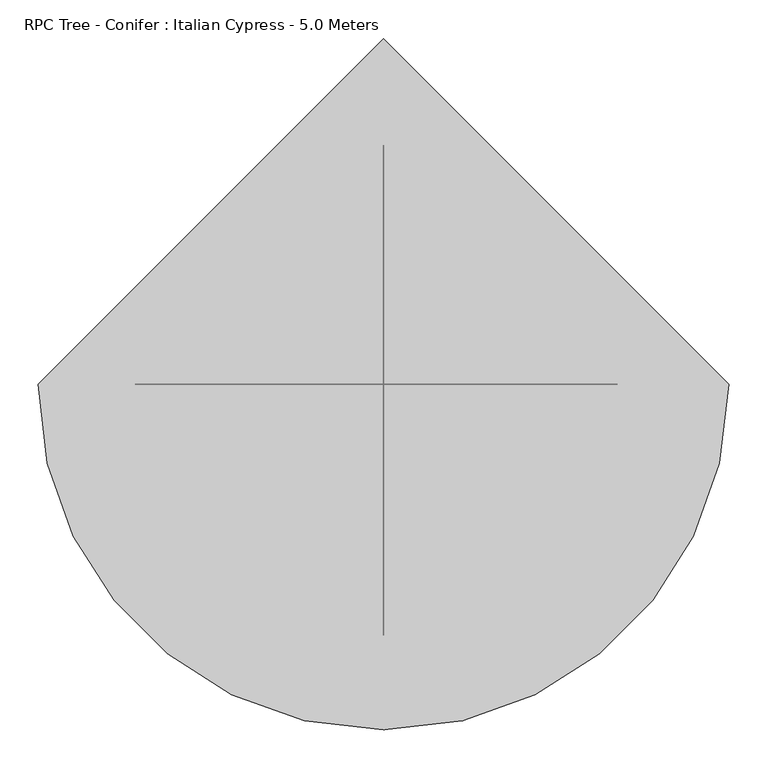
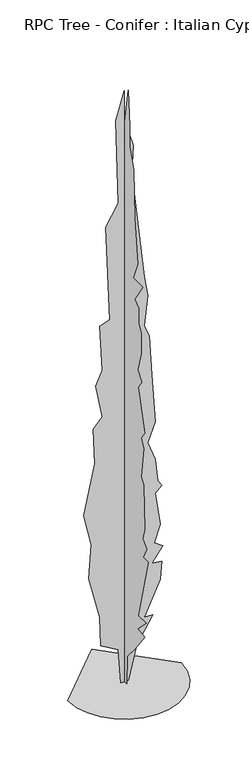
"""IFC4 building model written with IfcOpenShell, lengths in millimetres: geographic element geometry, RPC Tree - Conifer : Italian Cypress - 5.0 Meters."""

from ifc_helpers import new_model, si_unit, origin, place, context, project, spatial, triangles, source, transform, mapped, element, save


def rpc_tree_conifer_italian_cypress_5_0_meters_3d53936f(model_context):
    return source(origin(), model_context, "Body", "Tessellation", [
        triangles([(-28.9243291, 1.3e-06, 0.1175505), (-48.5995771, -1.5e-05, 287.7924989), (-186.3258362, -1.37e-05, 366.4949987), (-196.1633353, -2.79e-05, 612.4350014), (-284.7008453, -4.52e-05, 966.5875122), (-265.0258289, -6.24e-05, 1242.0400303), (-324.0508235, -7.57e-05, 1507.6550674), (-235.513586, -0.0001036, 1910.9949829), (-245.3513394, -0.0001208, 2206.1249336), (-176.4880827, -0.0001285, 2284.8250717), (-225.6760869, -0.0001427, 2560.275119), (-176.4880827, -0.0001519, 2678.3248901), (-196.1633353, -0.0001733, 3052.1500374), (-117.4625795, -0.0001785, 3081.6749794), (-146.9753311, -0.0002242, 3868.6749069), (-48.5993273, -0.0002384, 4035.9248726), (-68.2745799, -0.0002792, 4734.3749725), (0.5886036, -0.0002957, 4960.6501144), (0.5885936, -0.0002816, 4724.5499908), (69.4516701, -0.00027, 4478.5998871), (59.614171, -0.0002561, 4252.3500343), (157.9899204, -0.0002064, 3347.2750465), (187.5026721, -0.0001977, 3180.0500793), (157.9899204, -0.0001818, 2934.0999756), (197.3401711, -0.0001776, 2835.7248756), (217.0154055, -0.0001586, 2501.2499428), (246.5281571, -0.0001358, 2097.9100273), (187.5026721, -0.0001239, 1940.5100418), (246.5281571, -0.000117, 1783.1074402), (266.2041545, -0.0001068, 1596.1925411), (295.71667, -0.0001051, 1547.0049911), (246.5281571, -0.0001, 1497.8174412), (285.8791709, -8.53e-05, 1222.3650684), (236.690658, -7.5e-05, 1084.6375013), (305.5541691, -7.51e-05, 1035.450024), (217.0154055, -6.42e-05, 917.4000349), (295.71667, -6.7e-05, 907.5624813), (285.8791709, -5.78e-05, 759.997506), (157.9899204, -3.58e-05, 484.5449879), (226.8529046, -3.88e-05, 484.5449879), (98.9641719, -2.09e-05, 277.9549998), (30.1011696, -1.3e-06, 0.058986), (0.1966738, 26.4907499, 3.55e-05), (0.1966807, 16.6530749, 238.6054939), (0.196685, 95.3537455, 258.2800016), (0.196697, 203.5672438, 494.3825051), (0.1967129, 311.7799882, 819.0224642), (0.1967124, 233.0799954, 887.8875195), (0.1967188, 242.9174945, 1094.4749823), (0.1967282, 272.4299918, 1419.1174484), (0.1967333, 262.5924927, 1547.0049911), (0.1967324, 213.4047429, 1645.3799458), (0.1967414, 272.4299918, 1861.8074329), (0.1967478, 193.7295085, 2156.9350582), (0.196749, 174.0544922, 2274.9874454), (0.1967577, 223.242242, 2422.54995), (0.1967593, 164.2167569, 2658.6499283), (0.1967653, 174.054256, 2786.5499702), (0.1967665, 134.7039962, 2924.2749939), (0.1967759, 154.3792578, 3189.875061), (0.1967755, 85.5160011, 3317.775103), (0.1967853, 124.8664971, 3504.675032), (0.19679, 75.678502, 3799.8250397), (0.1967981, 36.3279992, 4094.9500488), (0.1968071, 65.8407486, 4340.8748634), (0.1968079, 26.4905001, 4468.7749054), (0.1968139, -3.0223, 4704.875029), (0.1968216, -52.2102488, 5000.0000381), (0.1968108, -71.8855014, 4704.875029), (0.1968066, -71.8855014, 4537.6250633), (0.1968002, -130.9109955, 4380.2250778), (0.1967852, -140.7485037, 3976.899987), (0.1967737, -180.0987453, 3612.9001122), (0.1967729, -121.0732512, 3465.3251083), (0.1967673, -248.962002, 3465.3251083), (0.1967647, -140.7485037, 3298.1001411), (0.1967635, -199.7739979, 3258.7499268), (0.1967579, -199.7739979, 3130.8498848), (0.1967536, -229.2867495, 3062.0000175), (0.1967493, -229.2867495, 2894.7500519), (0.1967472, -180.0987453, 2727.5250847), (0.1967416, -239.1242486, 2658.6499283), (0.1967438, -189.9364988, 2589.800061), (0.1967284, -278.475008, 2255.3124836), (0.1967275, -229.2867495, 2186.4499718), (0.1967259, -268.6375089, 2117.5849892), (0.1967195, -229.2867495, 1861.8074329), (0.1967156, -268.6375089, 1812.6200283), (0.1967054, -278.475008, 1448.6300365), (0.1967024, -248.9617477, 1350.2524658), (0.1966976, -307.9874871, 1301.0650612), (0.1966986, -258.7999917, 1202.6900339), (0.1966956, -327.6624853, 1202.6900339), (0.1966845, -189.9362444, 671.4600323), (0.1966797, -298.1500062, 671.4600323), (0.1966828, -180.0987453, 553.4074997), (0.1966781, -278.475008, 543.5699824), (0.196679, -150.5860028, 366.4949987), (0.1966781, -42.3724999, 238.6054939), (0.1966712, -32.534751, 3.2e-05), (-450.413314, 0.0, 5.36e-05), (-438.5008143, -103.2502475, 4.7e-05), (-404.5758139, -198.0692509, 3.98e-05), (-351.3483215, -281.7399977, 3.25e-05), (-281.5433345, -351.54751, 2.53e-05), (-197.8723334, -404.7699881, 1.85e-05), (-103.0535753, -438.6974957, 1.23e-05), (0.1966927, -450.6125024, 7.1e-06), (103.4469197, -438.6974957, 3.3e-06), (198.2659141, -404.7724952, 1.1e-06), (281.9366608, -351.5450028, 7e-07), (351.7441913, -281.7399977, 1.8e-06), (404.9666694, -198.0689966, 4.4e-06), (438.894177, -103.2502475, 8.6e-06), (450.8066766, 3.94e-05, 1.42e-05), (0.1966127, 450.6125024, 6.08e-05)], [[17, 18, 19], [39, 40, 41], [16, 17, 19], [16, 19, 20], [16, 20, 21], [16, 21, 22], [15, 16, 22], [14, 15, 22], [14, 22, 23], [14, 23, 24], [34, 35, 36], [36, 37, 38], [42, 1, 2], [41, 42, 2], [39, 41, 2], [30, 31, 32], [39, 2, 3], [39, 3, 4], [38, 39, 4], [36, 38, 4], [36, 4, 5], [34, 36, 5], [34, 5, 6], [33, 34, 6], [32, 33, 6], [32, 6, 7], [32, 7, 8], [30, 32, 8], [29, 30, 8], [28, 29, 8], [28, 8, 9], [27, 28, 9], [27, 9, 10], [26, 27, 10], [26, 10, 11], [26, 11, 12], [25, 26, 12], [25, 12, 13], [24, 25, 13], [14, 24, 13], [67, 68, 69], [94, 95, 96], [74, 75, 76], [96, 97, 98], [92, 93, 94], [100, 43, 44], [99, 100, 44], [67, 69, 70], [66, 67, 70], [66, 70, 71], [65, 66, 71], [65, 71, 72], [64, 65, 72], [63, 64, 72], [63, 72, 73], [62, 63, 73], [62, 73, 74], [61, 62, 74], [61, 74, 76], [90, 91, 92], [81, 82, 83], [46, 47, 48], [60, 61, 76], [59, 60, 76], [59, 76, 77], [59, 77, 78], [59, 78, 79], [59, 79, 80], [59, 80, 81], [58, 59, 81], [57, 58, 81], [57, 81, 83], [56, 57, 83], [56, 83, 84], [55, 56, 84], [55, 84, 85], [54, 55, 85], [53, 54, 85], [53, 85, 86], [53, 86, 87], [52, 53, 87], [52, 87, 88], [52, 88, 89], [51, 52, 89], [51, 89, 90], [50, 51, 90], [49, 50, 90], [49, 90, 92], [49, 92, 94], [48, 49, 94], [46, 48, 94], [46, 94, 96], [46, 96, 98], [45, 46, 98], [45, 98, 99], [44, 45, 99], [115, 116, 101], [114, 115, 101], [114, 101, 102], [113, 114, 102], [113, 102, 103], [113, 103, 104], [112, 113, 104], [111, 112, 104], [111, 104, 105], [111, 105, 106], [111, 106, 107], [111, 107, 108], [111, 108, 109], [111, 109, 110]], closed=False),
    ])


if __name__ == "__main__":
    model = new_model("IFC4")
    model_context = context("Model", 3, world=origin())
    ifc_project = project(units=[si_unit("LENGTHUNIT", "METRE", prefix="MILLI")], contexts=[model_context])
    site = spatial("IfcSite", under=ifc_project)
    building = spatial("IfcBuilding", under=site)
    placement = place(None, origin())
    rpc_tree_conifer_italian_cypress_5_0_meters_shape = rpc_tree_conifer_italian_cypress_5_0_meters_3d53936f(model_context)
    element("IfcGeographicElement", 1, ObjectType="RPC Tree - Conifer : Italian Cypress - 5.0 Meters", at=placement, inside=building, context=model_context, shape_type="MappedRepresentation", body=[
        mapped(rpc_tree_conifer_italian_cypress_5_0_meters_shape, transform((0.0, 0.0, 0.0), x_axis=(1.0, 0.0, 0.0), y_axis=(0.0, 1.0, 0.0), z_axis=(0.0, 0.0, 1.0))),
    ])
    save(model, "model.ifc")

# Revit data of these elements
# Type "RPC Tree - Conifer : Italian Cypress - 5.0 Meters"
#   built-in parameter 1005198 = "{2, 15},{39, RPC-16-FWM7-6P00-C8X0-C000-ST1L-LVER-AU},{1, 0},{1, 0},{2, 13},{1, 8},{5, Color},{1, 0},{1, 0},{3, 0.8},{3, 0.8},{3, 0.8},{1, 8},{7, BBoxMin},{1, 0},{1, 0},{1, 0},{1, 0},{1, 0},{1, 8},{7, BBoxMax},{1, 0},{1, 0},{1, 0},{1, 0},{1, 0},{2, 11},{9, RPCTypeId},{1, 0},{1, 0},{39, RPC-16-FWM7-6P00-C8X0-C000-ST1L-LVER-AU},{1, 6},{14, RPCPlantHeight},{1, 0},{1, 0},{7, 16.4042},{2, 11},{7, keyword},{1, 0},{1, 0},{34, :RPCs:Trees [General]:Geometry:RPC},{2, 11},{8, category},{1, 0},{1, 0},{15, Trees [General]},{2, 11},{12, LocalizedUID},{1, 0},{1, 0},{15, Italian Cypress},{2, 14},{6, Height},{1, 0},{1, 0},{7, 16.4042},{1, 2},{16, Cast Reflections},{1, 0},{1, 0},{1, 0},{1, 2},{12, Cast Shadows},{1, 0},{1, 0},{1, 1},{1, 2},{9, Lock View},{1, 0},{1, 0},{1, 0},{1, 4},{5, ViewC},{1, 0},{1, 0},{1, 0},{21, assetlibrary_base.fbx},{1, 5},"
#   built-in parameter 1005195 = "RPC-16-FWM7-6P00-C8X0-C000-ST1L-LVER-AU"
#   Type Comments = "Italian Cypress"
#   Height = 5000 mm
#   Description = (empty or 0)
#   Default Elevation = 0
